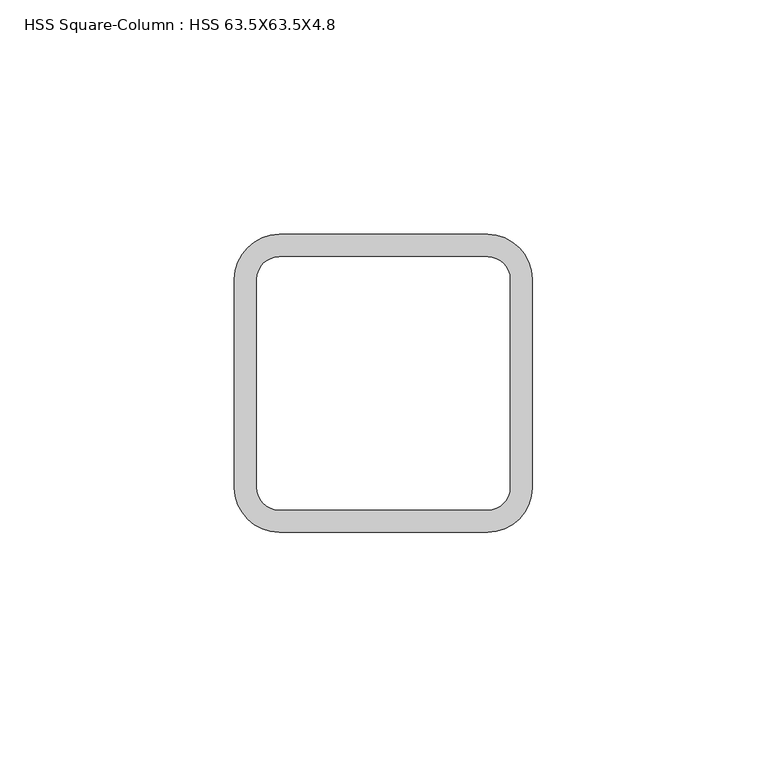
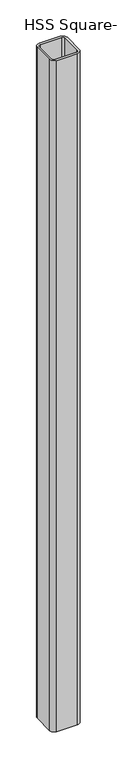
"""IFC4 building model written with IfcOpenShell, lengths in millimetres: column geometry, HSS Square-Column : HSS 63.5X63.5X4.8."""

from ifc_helpers import new_model, si_unit, point, frame, frame_2d, origin, place, context, project, spatial, polyline, circle_curve, trimmed, segment, composite_curve, outline, extrude, source, transform, mapped, element, save


def hss_square_column_hss_63_5x63_5x4_8_cb397b89(model_context):
    return source(origin(), model_context, "Body", "SweptSolid", [
        extrude(outline(composite_curve([segment(trimmed(circle_curve(frame_2d((22.225, 22.225)), 9.525), [point((22.225, 31.75))], [point((31.75, 22.225))], False, "CARTESIAN"), True, "CONTINUOUS"), segment(polyline([(31.75, 22.225), (31.75, -22.225)]), True, "CONTINUOUS"), segment(trimmed(circle_curve(frame_2d((22.225, -22.225)), 9.525), [point((31.75, -22.225))], [point((22.225, -31.75))], False, "CARTESIAN"), True, "CONTINUOUS"), segment(polyline([(22.225, -31.75), (-22.225, -31.75)]), True, "CONTINUOUS"), segment(trimmed(circle_curve(frame_2d((-22.225, -22.225)), 9.525), [point((-22.225, -31.75))], [point((-31.75, -22.225))], False, "CARTESIAN"), True, "CONTINUOUS"), segment(polyline([(-31.75, -22.225), (-31.75, 22.225)]), True, "CONTINUOUS"), segment(trimmed(circle_curve(frame_2d((-22.225, 22.225)), 9.525), [point((-31.75, 22.225))], [point((-22.225, 31.75))], False, "CARTESIAN"), True, "CONTINUOUS"), segment(polyline([(-22.225, 31.75), (22.225, 31.75)]), True, "CONTINUOUS")], self_intersect=False), holes=[composite_curve([segment(polyline([(22.225, 26.9875), (-22.225, 26.9875)]), True, "CONTINUOUS"), segment(trimmed(circle_curve(frame_2d((-22.225, 22.225)), 4.7625), [point((-22.225, 26.9875))], [point((-26.9875, 22.225))], True, "CARTESIAN"), True, "CONTINUOUS"), segment(polyline([(-26.9875, 22.225), (-26.9875, -22.225)]), True, "CONTINUOUS"), segment(trimmed(circle_curve(frame_2d((-22.225, -22.225)), 4.7625), [point((-26.9875, -22.225))], [point((-22.225, -26.9875))], True, "CARTESIAN"), True, "CONTINUOUS"), segment(polyline([(-22.225, -26.9875), (22.225, -26.9875)]), True, "CONTINUOUS"), segment(trimmed(circle_curve(frame_2d((22.225, -22.225)), 4.7625), [point((22.225, -26.9875))], [point((26.9875, -22.225))], True, "CARTESIAN"), True, "CONTINUOUS"), segment(polyline([(26.9875, -22.225), (26.9875, 22.225)]), True, "CONTINUOUS"), segment(trimmed(circle_curve(frame_2d((22.225, 22.225)), 4.7625), [point((26.9875, 22.225))], [point((22.225, 26.9875))], True, "CARTESIAN"), True, "CONTINUOUS")], self_intersect=False)]), frame((0.0, 0.0, 3220.0), z_axis=(0.0, 0.0, 1.0), x_axis=(1.0, 0.0, 0.0)), (0.0, 0.0, 1.0), 1500.0),
    ])


if __name__ == "__main__":
    model = new_model("IFC4")
    model_context = context("Model", 3, world=origin())
    ifc_project = project(units=[si_unit("LENGTHUNIT", "METRE", prefix="MILLI")], contexts=[model_context])
    site = spatial("IfcSite", under=ifc_project)
    building = spatial("IfcBuilding", under=site)
    placement = place(None, origin())
    hss_square_column_hss_63_5x63_5x4_8_shape = hss_square_column_hss_63_5x63_5x4_8_cb397b89(model_context)
    element("IfcColumn", 1, ObjectType="HSS Square-Column : HSS 63.5X63.5X4.8", at=placement, inside=building, context=model_context, shape_type="MappedRepresentation", body=[
        mapped(hss_square_column_hss_63_5x63_5x4_8_shape, transform((0.0, 0.0, 0.0), x_axis=(1.0, 0.0, 0.0), y_axis=(0.0, 1.0, 0.0), z_axis=(0.0, 0.0, 1.0))),
    ])
    save(model, "model.ifc")

# Revit data of these elements
# Type "HSS Square-Column : HSS 63.5X63.5X4.8"
#   Section Name Key = "HSS 2 1/2X2 1/2X3/16"
#   Assembly Code = "B10"
#   Width = 6.35 cm
#   Wall Nominal Thickness = 0.4763 cm
#   Wall Design Thickness = 0.442 cm
#   Torsional Moment of Inertia = 93.6521 cm⁴
#   Torsional Modulus = 30.4799 cm³
#   Section Area = 9.93546 cm²
#   Plastic Modulus weak axis = 21.6309 cm³
#   Plastic Modulus strong axis = 21.6309 cm³
#   Outer Fillet = 0.9525 cm
#   Nominal Weight = 8.31884 kgf/m
#   Moment of Inertia weak axis = 56.1912 cm⁴
#   Moment of Inertia strong axis = 56.1912 cm⁴
#   Inner Fillet = 0.4763 cm
#   Height = 6.35 cm
#   Elastic Modulus weak axis = 17.698 cm³
#   Elastic Modulus strong axis = 17.698 cm³
#   Centroid Vertical = 3.175 cm
#   Centroid Horizontal = 3.175 cm
#   Structural Material [instance default] = Steel ASTM A500, Grade B, Rectangular and Square
#   Principal Axes Angle = 0
# Element 1 (IfcColumn, "HSS Square-Column : HSS 63.5X63.5X4.8")
#   Structural Material = none
# Materials
#   "Steel ASTM A500, Grade B, Rectangular and Square": class "Metal", colour RGB 199 199 199, transparency 0, Description = "Carbon steel", Cost = 0
